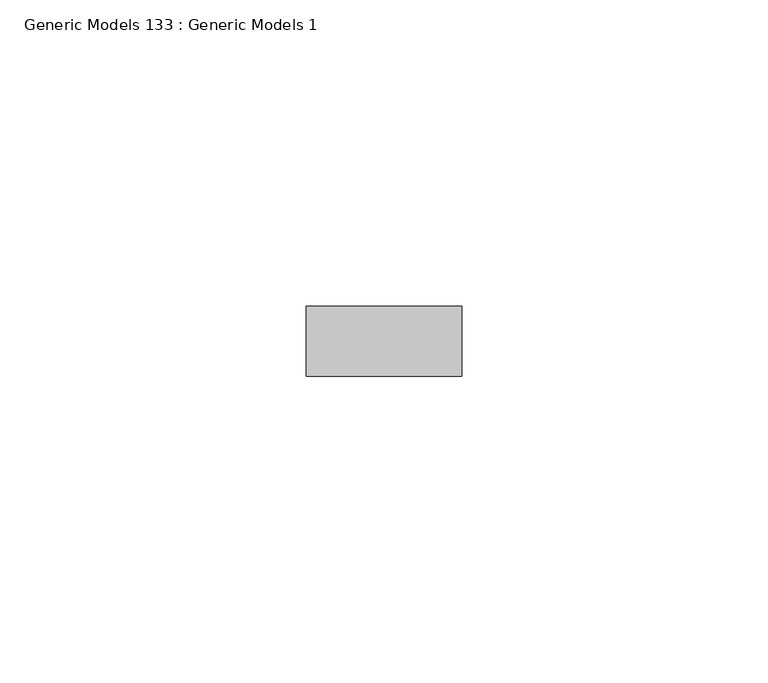
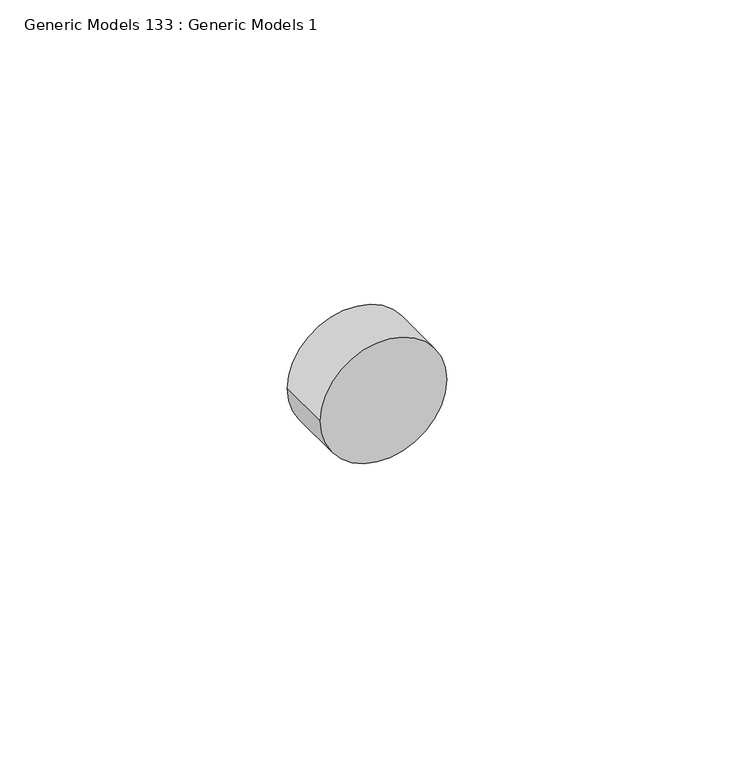
"""IFC4 building model written with IfcOpenShell, lengths in millimetres: proxy geometry, Generic Models 133 : Generic Models 1."""

from ifc_helpers import new_model, si_unit, point, frame, frame_2d, origin, place, context, project, spatial, circle_curve, trimmed, segment, composite_curve, outline, extrude, source, transform, mapped, element, save


def generic_models_133_generic_models_1_a35064e9(model_context):
    return source(origin(), model_context, "Body", "SweptSolid", [
        extrude(outline(composite_curve([segment(trimmed(circle_curve(frame_2d((38717.9805939, 8245.7828124)), 12.7), [point((38717.9805939, 8233.0828124))], [point((38717.9805939, 8258.4828124))], False, "CARTESIAN"), True, "CONTINUOUS"), segment(trimmed(circle_curve(frame_2d((38717.9805939, 8245.7828124)), 12.7), [point((38717.9805939, 8258.4828124))], [point((38717.9805939, 8233.0828124))], False, "CARTESIAN"), True, "CONTINUOUS")], self_intersect=False)), frame((0.0, 1836.9202358, 0.0), z_axis=(0.0, 1.0, 0.0), x_axis=(0.0, 0.0, 1.0)), (0.0, 0.0, 1.0), 11.4464372),
    ])


if __name__ == "__main__":
    model = new_model("IFC4")
    model_context = context("Model", 3, world=origin())
    ifc_project = project(units=[si_unit("LENGTHUNIT", "METRE", prefix="MILLI")], contexts=[model_context])
    site = spatial("IfcSite", under=ifc_project)
    building = spatial("IfcBuilding", under=site)
    placement = place(None, origin())
    generic_models_133_generic_models_1_shape = generic_models_133_generic_models_1_a35064e9(model_context)
    element("IfcBuildingElementProxy", 1, Name="Generic Models 133 : Generic Models 1", ObjectType="Generic Models 133 : Generic Models 1", at=placement, inside=building, context=model_context, shape_type="MappedRepresentation", body=[
        mapped(generic_models_133_generic_models_1_shape, transform((0.0, 0.0, 0.0), x_axis=(1.0, 0.0, 0.0), y_axis=(0.0, 1.0, 0.0), z_axis=(0.0, 0.0, 1.0))),
    ])
    save(model, "model.ifc")

# Revit data of these elements
# Element 1 (IfcBuildingElementProxy, "Generic Models 133 : Generic Models 1")
#   Materials on its faces: "S.S. LAG BOLT - SEE STRUCT. DWGS"
# Materials
#   "S.S. LAG BOLT - SEE STRUCT. DWGS": class "Generic", colour RGB 120 120 120, transparency 0, Cost = 0
